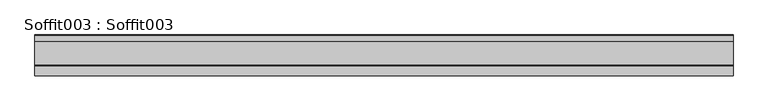
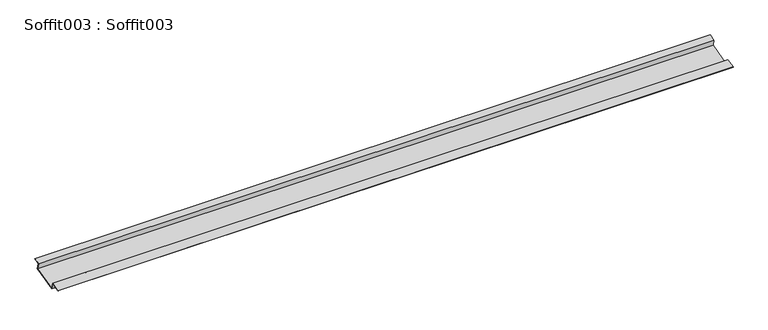
"""IFC4 building model written with IfcOpenShell, lengths in millimetres: proxy geometry, Soffit003 : Soffit003."""

from ifc_helpers import new_model, si_unit, frame, origin, place, context, project, spatial, polyline, outline, extrude, source, transform, mapped, element, save


def soffit003_soffit003_57078732(model_context):
    return source(origin(), model_context, "Body", "SweptSolid", [
        extrude(outline(polyline([(-5244.0236011, 42427.9124632), (-5239.3852349, 42409.3953515), (-5313.3015493, 42390.8799942), (-5317.9399151, 42409.4022563), (-5343.409089, 42403.024237), (-5343.7175976, 42404.2561958), (-5317.0164648, 42410.9427236), (-5312.3781193, 42392.4205423), (-5240.9257627, 42410.3187007), (-5245.5641492, 42428.8358932), (-5227.0077672, 42433.4828034), (-5226.6992587, 42432.2508446), (-5244.0236011, 42427.9124632)])), frame((12382.7678845, 0.0, 0.0), z_axis=(1.0, 0.0, 0.0), x_axis=(0.0, 1.0, 0.0)), (0.0, 0.0, 1.0), 2000.25),
    ])


if __name__ == "__main__":
    model = new_model("IFC4")
    model_context = context("Model", 3, world=origin())
    ifc_project = project(units=[si_unit("LENGTHUNIT", "METRE", prefix="MILLI")], contexts=[model_context])
    site = spatial("IfcSite", under=ifc_project)
    building = spatial("IfcBuilding", under=site)
    placement = place(None, origin())
    soffit003_soffit003_shape = soffit003_soffit003_57078732(model_context)
    element("IfcBuildingElementProxy", 1, Name="Soffit003 : Soffit003", ObjectType="Soffit003 : Soffit003", at=placement, inside=building, context=model_context, shape_type="MappedRepresentation", body=[
        mapped(soffit003_soffit003_shape, transform((0.0, 0.0, 0.0), x_axis=(1.0, 0.0, 0.0), y_axis=(0.0, 1.0, 0.0), z_axis=(0.0, 0.0, 1.0))),
    ])
    save(model, "model.ifc")

# Revit data of these elements
# Type "Soffit003 : Soffit003"
#   NameOverride = "Soffit003"
# Element 1 (IfcBuildingElementProxy, "Soffit003 : Soffit003")
#   Materials on its faces: "16 GA. COPPER SOFFIT DRIP SCREED"
# Materials
#   "16 GA. COPPER SOFFIT DRIP SCREED": class "Unassigned", colour RGB 255 217 0, transparency 0
